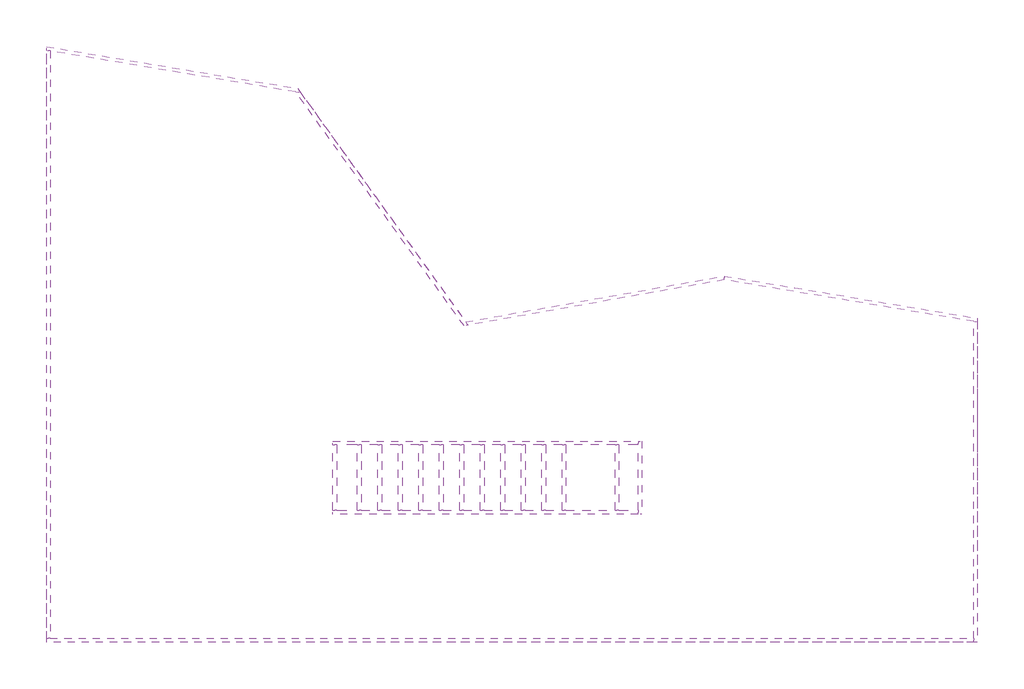
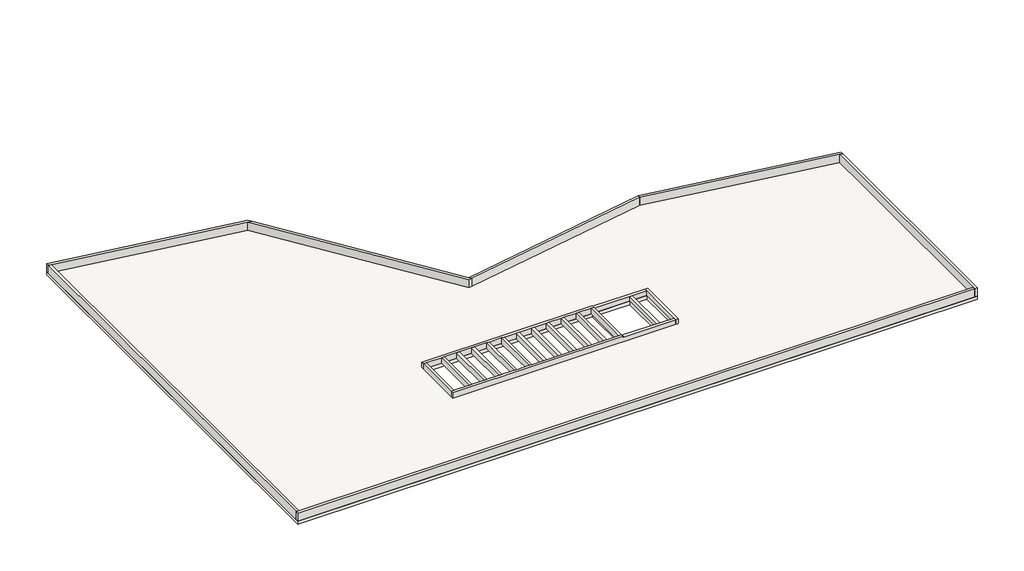
# One storey: 23 walls, 1 slab.
"""IFC4 building model written with IfcOpenShell, lengths in millimetres."""

from ifc_helpers import new_model, si_unit, frame, origin, place, context, project, spatial, polyline, outline, extrude, faceted_brep, element, save

model = new_model("IFC4")

# Units and contexts
model_context = context("Model", 3, world=origin())
ifc_project = project(units=[si_unit("LENGTHUNIT", "METRE", prefix="MILLI")], contexts=[model_context])

# Site, building, storey
site = spatial("IfcSite", under=ifc_project)
building = spatial("IfcBuilding", under=site)
storey = spatial("IfcBuildingStorey", under=building, Name="04_OG_OKFB_13,84", Elevation=13840.0)

# Slab
placement = place(None, origin())
element("IfcSlab", 1, ObjectType="5dki Decke Ortbeton 25cm C30/37_f", at=placement, inside=storey, context=model_context, shape_type="SweptSolid", body=[
    extrude(outline(polyline([(-129.9989953, 31855.7150729), (13359.8955383, 29603.0549033), (22383.5041721, 17069.4128529), (36259.9888873, 19532.5499737), (49863.9990833, 17260.8337794), (49863.9991105, -129.9989509), (-129.9989953, -129.9990284), (-129.9989953, 31855.7150729)]), holes=[polyline([(27641.9999883, 10442.0127204), (15367.0008797, 10442.0127204), (15367.0008797, 6960.0000464), (27641.9999883, 6960.0000464), (27641.9999883, 10442.0127204)]), polyline([(27891.9992024, 6990.0014141), (30391.5781103, 6990.0014141), (30391.5781103, 10412.0125176), (27891.9992024, 10412.0125176), (27891.9992024, 6990.0014141)]), polyline([(30635.8205887, 6960.0014903), (31641.9991143, 6960.0014903), (31641.9991143, 10412.0130303), (30635.8205887, 10412.0130303), (30635.8205887, 6960.0014903)])]), frame((0.0, 0.0, 16900.0), z_axis=(0.0, 0.0, 1.0), x_axis=(1.0, 0.0, 0.0)), (0.0, 0.0, 1.0), 250.0),
])

# Walls
element("IfcWall", 2, ObjectType="5dki Unterzug 20cm C25/30", at=placement, inside=storey, context=model_context, shape_type="Brep", body=[
    faceted_brep([(-130.0001888, 31652.9459223, 17150.0), (69.9998112, 31619.548179, 17150.0), (13245.710804, 29419.3531156, 17150.0), (13525.8286333, 29372.5765989, 17150.0), (13525.8286333, 29372.5765989, 17780.0), (13245.710804, 29419.3531156, 17780.0), (69.9998112, 31619.548179, 17780.0), (-130.0001888, 31652.9459223, 17780.0), (-130.0001888, 31855.7152722, 17150.0), (-130.0001888, 31855.7152722, 17780.0), (13359.8955383, 29603.0549033, 17780.0), (13359.8955383, 29603.0549033, 17150.0)], [[[0, 1, 2, 3, 4, 5, 6, 7]], [[8, 9, 10, 11]], [[3, 2, 1, 0, 8, 11]], [[7, 6, 5, 4, 10, 9]], [[4, 3, 11, 10]], [[0, 7, 9, 8]]]),
])
element("IfcWall", 3, ObjectType="5dki Unterzug 20cm C25/30", at=placement, inside=storey, context=model_context, shape_type="Brep", body=[
    faceted_brep([(13245.710804, 29419.3531156, 17150.0), (22294.6581946, 16850.5159542, 17150.0), (22294.6581946, 16850.5159542, 17780.0), (13245.710804, 29419.3531156, 17780.0), (13525.8286333, 29372.5765989, 17150.0), (13525.8286333, 29372.5765989, 17780.0), (22383.5041721, 17069.4128529, 17780.0), (22513.1740957, 16889.3034894, 17780.0), (22513.1740957, 16889.3034894, 17150.0), (22383.5041721, 17069.4128529, 17150.0)], [[[0, 1, 2, 3]], [[4, 5, 6, 7, 8, 9]], [[1, 0, 4, 9, 8]], [[3, 2, 7, 6, 5]], [[0, 3, 5, 4]], [[2, 1, 8, 7]]]),
])
element("IfcWall", 4, ObjectType="5dki Unterzug 20cm C25/30", at=placement, inside=storey, context=model_context, shape_type="SweptSolid", body=[
    extrude(outline(polyline([(36260.2920068, 19329.4774895), (22513.1740957, 16889.3034894), (22383.5041721, 17069.4128529), (36259.255712, 19532.4198889), (36260.2920068, 19329.4774895)])), frame((0.0, 0.0, 17150.0), z_axis=(0.0, 0.0, 1.0), x_axis=(1.0, 0.0, 0.0)), (0.0, 0.0, 1.0), 630.0),
])
element("IfcWall", 5, ObjectType="5dki Unterzug 20cm C25/30", at=placement, inside=storey, context=model_context, shape_type="Brep", body=[
    faceted_brep([(36260.2920068, 19329.4774895, 17150.0), (49663.9990837, 17091.2096558, 17150.0), (49863.9990837, 17057.8119126, 17150.0), (49863.9990837, 17057.8119126, 17780.0), (49663.9990837, 17091.2096558, 17780.0), (36260.2920068, 19329.4774895, 17780.0), (36259.255712, 19532.4198889, 17150.0), (36259.255712, 19532.4198889, 17780.0), (49863.9990834, 17260.5812626, 17780.0), (49863.9990834, 17260.5812626, 17150.0)], [[[0, 1, 2, 3, 4, 5]], [[6, 7, 8, 9]], [[2, 1, 0, 6, 9]], [[5, 4, 3, 8, 7]], [[0, 5, 7, 6]], [[3, 2, 9, 8]]]),
])
element("IfcWall", 6, ObjectType="5dki Unterzug 20cm C25/30", at=placement, inside=storey, context=model_context, shape_type="Brep", body=[
    faceted_brep([(49663.9990837, 17091.2096558, 17150.0), (49663.9991102, 70.0010491, 17150.0), (49663.9991105, -129.9989509, 17150.0), (49663.9991105, -129.9989509, 17780.0), (49663.9991102, 70.0010491, 17780.0), (49663.9990837, 17091.2096558, 17780.0), (49863.9990837, 17057.8119126, 17150.0), (49863.9990837, 17057.8119126, 17780.0), (49863.9991105, -129.9989509, 17780.0), (49863.9991105, -129.9989509, 17150.0)], [[[0, 1, 2, 3, 4, 5]], [[6, 7, 8, 9]], [[2, 1, 0, 6, 9]], [[5, 4, 3, 8, 7]], [[0, 5, 7, 6]], [[3, 2, 9, 8]]]),
])
element("IfcWall", 7, ObjectType="5dki Unterzug 20cm C25/30", at=placement, inside=storey, context=model_context, shape_type="Brep", body=[
    faceted_brep([(49663.9991102, 70.0010491, 17150.0), (69.9998112, 70.0010491, 17150.0), (-130.0001888, 70.0010491, 17150.0), (-130.0001888, 70.0010491, 17780.0), (69.9998112, 70.0010491, 17780.0), (49663.9991102, 70.0010491, 17780.0), (49663.9991105, -129.9989509, 17150.0), (49663.9991105, -129.9989509, 17780.0), (-130.0001888, -129.9989509, 17780.0), (-130.0001888, -129.9989509, 17150.0)], [[[0, 1, 2, 3, 4, 5]], [[6, 7, 8, 9]], [[2, 1, 0, 6, 9]], [[5, 4, 3, 8, 7]], [[0, 5, 7, 6]], [[3, 2, 9, 8]]]),
])
element("IfcWall", 8, ObjectType="5dki Unterzug 20cm C25/30", at=placement, inside=storey, context=model_context, shape_type="SweptSolid", body=[
    extrude(outline(polyline([(69.9998112, 31619.548179), (69.9998112, 70.0010491), (-130.0001888, 70.0010491), (-130.0001888, 31652.9459223), (69.9998112, 31619.548179)])), frame((0.0, 0.0, 17150.0), z_axis=(0.0, 0.0, 1.0), x_axis=(1.0, 0.0, 0.0)), (0.0, 0.0, 1.0), 630.0),
])
element("IfcWall", 9, ObjectType="5dki Überzug 20cm C30/37", at=placement, inside=storey, context=model_context, shape_type="Brep", body=[
    faceted_brep([(15242.0008797, 10462.0127204, 17150.0), (16566.9999827, 10462.0127204, 17150.0), (16766.9999827, 10462.0127204, 17150.0), (17666.9999827, 10462.0127204, 17150.0), (17866.9999827, 10462.0127204, 17150.0), (18766.9999827, 10462.0127204, 17150.0), (18966.9999827, 10462.0127204, 17150.0), (19866.9999827, 10462.0127204, 17150.0), (20066.9999827, 10462.0127204, 17150.0), (20966.9999827, 10462.0127204, 17150.0), (21166.9999827, 10462.0127204, 17150.0), (22066.9999827, 10462.0127204, 17150.0), (22266.9999827, 10462.0127204, 17150.0), (23166.9999827, 10462.0127204, 17150.0), (23366.9999827, 10462.0127204, 17150.0), (24266.9999827, 10462.0127204, 17150.0), (24466.9999827, 10462.0127204, 17150.0), (25366.9999827, 10462.0127204, 17150.0), (25566.9999827, 10462.0127204, 17150.0), (26466.9999827, 10462.0127204, 17150.0), (26666.9999827, 10462.0127204, 17150.0), (27566.9999827, 10462.0127204, 17150.0), (27766.9999827, 10462.0127204, 17150.0), (30401.9991143, 10462.0127204, 17150.0), (30601.9991143, 10462.0127204, 17150.0), (31641.9991143, 10462.0127204, 17150.0), (31641.9991143, 10462.0127204, 17530.0), (27766.9999827, 10462.0127204, 17530.0), (27766.9999827, 10462.0127204, 17580.0), (27566.9999827, 10462.0127204, 17580.0), (26666.9999827, 10462.0127204, 17580.0), (26466.9999827, 10462.0127204, 17580.0), (25566.9999827, 10462.0127204, 17580.0), (25366.9999827, 10462.0127204, 17580.0), (24466.9999827, 10462.0127204, 17580.0), (24266.9999827, 10462.0127204, 17580.0), (23366.9999827, 10462.0127204, 17580.0), (23166.9999827, 10462.0127204, 17580.0), (22266.9999827, 10462.0127204, 17580.0), (22066.9999827, 10462.0127204, 17580.0), (21166.9999827, 10462.0127204, 17580.0), (20966.9999827, 10462.0127204, 17580.0), (20066.9999827, 10462.0127204, 17580.0), (19866.9999827, 10462.0127204, 17580.0), (18966.9999827, 10462.0127204, 17580.0), (18766.9999827, 10462.0127204, 17580.0), (17866.9999827, 10462.0127204, 17580.0), (17666.9999827, 10462.0127204, 17580.0), (16766.9999827, 10462.0127204, 17580.0), (16566.9999827, 10462.0127204, 17580.0), (15442.0008797, 10462.0127204, 17580.0), (15242.0008797, 10462.0127204, 17580.0), (15242.0008797, 10662.0127204, 17150.0), (15242.0008797, 10662.0127204, 17580.0), (27766.9999827, 10662.0127204, 17580.0), (27766.9999827, 10662.0127204, 17530.0), (31641.9991143, 10662.0127204, 17530.0), (31641.9991143, 10662.0127204, 17150.0)], [[[0, 1, 2, 3, 4, 5, 6, 7, 8, 9, 10, 11, 12, 13, 14, 15, 16, 17, 18, 19, 20, 21, 22, 23, 24, 25, 26, 27, 28, 29, 30, 31, 32, 33, 34, 35, 36, 37, 38, 39, 40, 41, 42, 43, 44, 45, 46, 47, 48, 49, 50, 51]], [[52, 53, 54, 55, 56, 57]], [[0, 51, 53, 52]], [[26, 25, 57, 56]], [[25, 24, 23, 22, 21, 20, 19, 18, 17, 16, 15, 14, 13, 12, 11, 10, 9, 8, 7, 6, 5, 4, 3, 2, 1, 0, 52, 57]], [[27, 26, 56, 55]], [[51, 50, 49, 48, 47, 46, 45, 44, 43, 42, 41, 40, 39, 38, 37, 36, 35, 34, 33, 32, 31, 30, 29, 28, 54, 53]], [[28, 27, 55, 54]]]),
])
element("IfcWall", 10, ObjectType="5dki Überzug 20cm C30/37", at=placement, inside=storey, context=model_context, shape_type="Brep", body=[
    faceted_brep([(27566.9999827, 10462.0127204, 17580.0), (27566.9999827, 10462.0127204, 17150.0), (27566.9999827, 6940.0000311, 17150.0), (27566.9999827, 6940.0000311, 17580.0), (27766.9999827, 10462.0127204, 17150.0), (27766.9999827, 10462.0127204, 17530.0), (27766.9999827, 10462.0127204, 17580.0), (27766.9999827, 6940.0000311, 17580.0), (27766.9999827, 6940.0000311, 17530.0), (27766.9999827, 6940.0000311, 17150.0)], [[[0, 1, 2, 3]], [[4, 5, 6, 7, 8, 9]], [[2, 1, 4, 9]], [[0, 3, 7, 6]], [[0, 6, 5, 4, 1]], [[3, 2, 9, 8, 7]]]),
])
element("IfcWall", 11, ObjectType="5dki Überzug 20cm C30/37", at=placement, inside=storey, context=model_context, shape_type="Brep", body=[
    faceted_brep([(15242.0008797, 6940.0000311, 17150.0), (15242.0008797, 6940.0000311, 17580.0), (15442.0008797, 6940.0000311, 17580.0), (16566.9999827, 6940.0000311, 17580.0), (16766.9999827, 6940.0000311, 17580.0), (17666.9999827, 6940.0000311, 17580.0), (17866.9999827, 6940.0000311, 17580.0), (18766.9999827, 6940.0000311, 17580.0), (18966.9999827, 6940.0000311, 17580.0), (19866.9999827, 6940.0000311, 17580.0), (20066.9999827, 6940.0000311, 17580.0), (20966.9999827, 6940.0000311, 17580.0), (21166.9999827, 6940.0000311, 17580.0), (22066.9999827, 6940.0000311, 17580.0), (22266.9999827, 6940.0000311, 17580.0), (23166.9999827, 6940.0000311, 17580.0), (23366.9999827, 6940.0000311, 17580.0), (24266.9999827, 6940.0000311, 17580.0), (24466.9999827, 6940.0000311, 17580.0), (25366.9999827, 6940.0000311, 17580.0), (25566.9999827, 6940.0000311, 17580.0), (26466.9999827, 6940.0000311, 17580.0), (26666.9999827, 6940.0000311, 17580.0), (27566.9999827, 6940.0000311, 17580.0), (27766.9999827, 6940.0000311, 17580.0), (27766.9999827, 6940.0000311, 17530.0), (31641.9991143, 6940.0000311, 17530.0), (31641.9991143, 6940.0000311, 17150.0), (30601.9991143, 6940.0000311, 17150.0), (30401.9991143, 6940.0000311, 17150.0), (27766.9999827, 6940.0000311, 17150.0), (27566.9999827, 6940.0000311, 17150.0), (26666.9999827, 6940.0000311, 17150.0), (26466.9999827, 6940.0000311, 17150.0), (25566.9999827, 6940.0000311, 17150.0), (25366.9999827, 6940.0000311, 17150.0), (24466.9999827, 6940.0000311, 17150.0), (24266.9999827, 6940.0000311, 17150.0), (23366.9999827, 6940.0000311, 17150.0), (23166.9999827, 6940.0000311, 17150.0), (22266.9999827, 6940.0000311, 17150.0), (22066.9999827, 6940.0000311, 17150.0), (21166.9999827, 6940.0000311, 17150.0), (20966.9999827, 6940.0000311, 17150.0), (20066.9999827, 6940.0000311, 17150.0), (19866.9999827, 6940.0000311, 17150.0), (18966.9999827, 6940.0000311, 17150.0), (18766.9999827, 6940.0000311, 17150.0), (17866.9999827, 6940.0000311, 17150.0), (17666.9999827, 6940.0000311, 17150.0), (16766.9999827, 6940.0000311, 17150.0), (16566.9999827, 6940.0000311, 17150.0), (15242.0008797, 6740.0000311, 17150.0), (31641.9991143, 6740.0000311, 17150.0), (31641.9991143, 6740.0000311, 17530.0), (27766.9999827, 6740.0000311, 17530.0), (27766.9999827, 6740.0000311, 17580.0), (15242.0008797, 6740.0000311, 17580.0)], [[[0, 1, 2, 3, 4, 5, 6, 7, 8, 9, 10, 11, 12, 13, 14, 15, 16, 17, 18, 19, 20, 21, 22, 23, 24, 25, 26, 27, 28, 29, 30, 31, 32, 33, 34, 35, 36, 37, 38, 39, 40, 41, 42, 43, 44, 45, 46, 47, 48, 49, 50, 51]], [[52, 53, 54, 55, 56, 57]], [[1, 0, 52, 57]], [[0, 51, 50, 49, 48, 47, 46, 45, 44, 43, 42, 41, 40, 39, 38, 37, 36, 35, 34, 33, 32, 31, 30, 29, 28, 27, 53, 52]], [[24, 23, 22, 21, 20, 19, 18, 17, 16, 15, 14, 13, 12, 11, 10, 9, 8, 7, 6, 5, 4, 3, 2, 1, 57, 56]], [[26, 25, 55, 54]], [[27, 26, 54, 53]], [[25, 24, 56, 55]]]),
])
element("IfcWall", 12, ObjectType="5dki Überzug 20cm C30/37", at=placement, inside=storey, context=model_context, shape_type="Brep", body=[
    faceted_brep([(15442.0008797, 6940.0000311, 16900.0), (15442.0008797, 10462.0127204, 16900.0), (15442.0008797, 10462.0127204, 17580.0), (15442.0008797, 6940.0000311, 17580.0), (15242.0008797, 6940.0000311, 16900.0), (15242.0008797, 6940.0000311, 17150.0), (15242.0008797, 6940.0000311, 17580.0), (15242.0008797, 10462.0127204, 17580.0), (15242.0008797, 10462.0127204, 17150.0), (15242.0008797, 10462.0127204, 16900.0)], [[[0, 1, 2, 3]], [[4, 5, 6, 7, 8, 9]], [[1, 0, 4, 9]], [[3, 2, 7, 6]], [[2, 1, 9, 8, 7]], [[0, 3, 6, 5, 4]]]),
])
element("IfcWall", 13, ObjectType="5dki Überzug 20cm C30/37", at=placement, inside=storey, context=model_context, shape_type="Brep", body=[
    faceted_brep([(31641.9991143, 10662.0127204, 17150.0), (31641.9991143, 10462.0127204, 17150.0), (31641.9991143, 6940.0000311, 17150.0), (31641.9991143, 6740.0000311, 17150.0), (31641.9991143, 6740.0000311, 17530.0), (31641.9991143, 6940.0000311, 17530.0), (31641.9991143, 10462.0127204, 17530.0), (31641.9991143, 10662.0127204, 17530.0), (31841.9991143, 10662.0127204, 17150.0), (31841.9991143, 10662.0127204, 17530.0), (31841.9991143, 6740.0000311, 17530.0), (31841.9991143, 6740.0000311, 17150.0)], [[[0, 1, 2, 3, 4, 5, 6, 7]], [[8, 9, 10, 11]], [[4, 3, 11, 10]], [[0, 7, 9, 8]], [[3, 2, 1, 0, 8, 11]], [[7, 6, 5, 4, 10, 9]]]),
])
element("IfcWall", 14, ObjectType="5dki Überzug 20cm C30/37", at=placement, inside=storey, context=model_context, shape_type="SweptSolid", body=[
    extrude(outline(polyline([(30401.9991143, 6940.0000311), (30401.9991143, 10462.0127204), (30601.9991143, 10462.0127204), (30601.9991143, 6940.0000311), (30401.9991143, 6940.0000311)])), frame((0.0, 0.0, 17150.0), z_axis=(0.0, 0.0, 1.0), x_axis=(1.0, 0.0, 0.0)), (0.0, 0.0, 1.0), 350.0),
])
element("IfcWall", 15, ObjectType="5dki Überzug 20cm C30/37", at=placement, inside=storey, context=model_context, shape_type="SweptSolid", body=[
    extrude(outline(polyline([(26466.9999827, 6940.0000311), (26466.9999827, 10462.0127204), (26666.9999827, 10462.0127204), (26666.9999827, 6940.0000311), (26466.9999827, 6940.0000311)])), frame((0.0, 0.0, 17150.0), z_axis=(0.0, 0.0, 1.0), x_axis=(1.0, 0.0, 0.0)), (0.0, 0.0, 1.0), 430.0),
])
element("IfcWall", 16, ObjectType="5dki Überzug 20cm C30/37", at=placement, inside=storey, context=model_context, shape_type="SweptSolid", body=[
    extrude(outline(polyline([(25366.9999827, 6940.0000311), (25366.9999827, 10462.0127204), (25566.9999827, 10462.0127204), (25566.9999827, 6940.0000311), (25366.9999827, 6940.0000311)])), frame((0.0, 0.0, 17150.0), z_axis=(0.0, 0.0, 1.0), x_axis=(1.0, 0.0, 0.0)), (0.0, 0.0, 1.0), 430.0),
])
element("IfcWall", 17, ObjectType="5dki Überzug 20cm C30/37", at=placement, inside=storey, context=model_context, shape_type="SweptSolid", body=[
    extrude(outline(polyline([(24266.9999827, 6940.0000311), (24266.9999827, 10462.0127204), (24466.9999827, 10462.0127204), (24466.9999827, 6940.0000311), (24266.9999827, 6940.0000311)])), frame((0.0, 0.0, 17150.0), z_axis=(0.0, 0.0, 1.0), x_axis=(1.0, 0.0, 0.0)), (0.0, 0.0, 1.0), 430.0),
])
element("IfcWall", 18, ObjectType="5dki Überzug 20cm C30/37", at=placement, inside=storey, context=model_context, shape_type="SweptSolid", body=[
    extrude(outline(polyline([(23166.9999827, 6940.0000311), (23166.9999827, 10462.0127204), (23366.9999827, 10462.0127204), (23366.9999827, 6940.0000311), (23166.9999827, 6940.0000311)])), frame((0.0, 0.0, 17150.0), z_axis=(0.0, 0.0, 1.0), x_axis=(1.0, 0.0, 0.0)), (0.0, 0.0, 1.0), 430.0),
])
element("IfcWall", 19, ObjectType="5dki Überzug 20cm C30/37", at=placement, inside=storey, context=model_context, shape_type="SweptSolid", body=[
    extrude(outline(polyline([(22066.9999827, 6940.0000311), (22066.9999827, 10462.0127204), (22266.9999827, 10462.0127204), (22266.9999827, 6940.0000311), (22066.9999827, 6940.0000311)])), frame((0.0, 0.0, 17150.0), z_axis=(0.0, 0.0, 1.0), x_axis=(1.0, 0.0, 0.0)), (0.0, 0.0, 1.0), 430.0),
])
element("IfcWall", 20, ObjectType="5dki Überzug 20cm C30/37", at=placement, inside=storey, context=model_context, shape_type="SweptSolid", body=[
    extrude(outline(polyline([(20966.9999827, 6940.0000311), (20966.9999827, 10462.0127204), (21166.9999827, 10462.0127204), (21166.9999827, 6940.0000311), (20966.9999827, 6940.0000311)])), frame((0.0, 0.0, 17150.0), z_axis=(0.0, 0.0, 1.0), x_axis=(1.0, 0.0, 0.0)), (0.0, 0.0, 1.0), 430.0),
])
element("IfcWall", 21, ObjectType="5dki Überzug 20cm C30/37", at=placement, inside=storey, context=model_context, shape_type="SweptSolid", body=[
    extrude(outline(polyline([(19866.9999827, 6940.0000311), (19866.9999827, 10462.0127204), (20066.9999827, 10462.0127204), (20066.9999827, 6940.0000311), (19866.9999827, 6940.0000311)])), frame((0.0, 0.0, 17150.0), z_axis=(0.0, 0.0, 1.0), x_axis=(1.0, 0.0, 0.0)), (0.0, 0.0, 1.0), 430.0),
])
element("IfcWall", 22, ObjectType="5dki Überzug 20cm C30/37", at=placement, inside=storey, context=model_context, shape_type="SweptSolid", body=[
    extrude(outline(polyline([(18766.9999827, 6940.0000311), (18766.9999827, 10462.0127204), (18966.9999827, 10462.0127204), (18966.9999827, 6940.0000311), (18766.9999827, 6940.0000311)])), frame((0.0, 0.0, 17150.0), z_axis=(0.0, 0.0, 1.0), x_axis=(1.0, 0.0, 0.0)), (0.0, 0.0, 1.0), 430.0),
])
element("IfcWall", 23, ObjectType="5dki Überzug 20cm C30/37", at=placement, inside=storey, context=model_context, shape_type="SweptSolid", body=[
    extrude(outline(polyline([(17666.9999827, 6940.0000311), (17666.9999827, 10462.0127204), (17866.9999827, 10462.0127204), (17866.9999827, 6940.0000311), (17666.9999827, 6940.0000311)])), frame((0.0, 0.0, 17150.0), z_axis=(0.0, 0.0, 1.0), x_axis=(1.0, 0.0, 0.0)), (0.0, 0.0, 1.0), 430.0),
])
element("IfcWall", 24, ObjectType="5dki Überzug 20cm C30/37", at=placement, inside=storey, context=model_context, shape_type="SweptSolid", body=[
    extrude(outline(polyline([(16566.9999827, 6940.0000311), (16566.9999827, 10462.0127204), (16766.9999827, 10462.0127204), (16766.9999827, 6940.0000311), (16566.9999827, 6940.0000311)])), frame((0.0, 0.0, 17150.0), z_axis=(0.0, 0.0, 1.0), x_axis=(1.0, 0.0, 0.0)), (0.0, 0.0, 1.0), 430.0),
])

save(model, "model.ifc")

# Revit data of these elements
# Type "5dki Decke Ortbeton 25cm C30/37_f"
#   cpiComponentType = "Slab"
#   cpiFitMatchKey = ""
#   5d Materialgüte = "C30/37"
#   Function = 0
#   5dki WU = no
#   Layers, outside or top first: 0.250 m "5d Beton - Stahlbeton" (function 1)
# Type "5dki Unterzug 20cm C25/30"
#   Type Comments = ""
#   Description = ""
#   cpiComponentType = "Beam"
#   cpiFitMatchKey = "5D-KI-STB-OB-TR-UZ"
#   5d Materialgüte = "C25/30"
#   Filter Tragend / Nichttragend = yes
#   5dki WU = no
#   Layers, outside or top first: 0.200 m "5d Beton - Stahlbeton" (function 1)
# Type "5dki Überzug 20cm C30/37"
#   Type Comments = ""
#   Description = ""
#   cpiComponentType = "Beam"
#   cpiFitMatchKey = "5D-KI-STB-OB-TR-UEZ"
#   5d Materialgüte = "C30/37"
#   Filter Tragend / Nichttragend = yes
#   Layers, outside or top first: 0.200 m "5d Beton - Stahlbeton" (function 1)
# Element 1 (IfcSlab, "5dki Decke Ortbeton 25cm C30/37_f")
#   000_080_030_Geschoß = "04_OG"
#   built-in parameter 1001955 = 2.97613 (stored number, unit not read)
#   Height Offset From Level = 0.000 m
#   built-in parameter 1001954 = 1
#   Phase Created = Neu
#   Materials on its faces: "5d Beton - Stahlbeton"
# Elements 2, 3, 4, 5, 6, 7, 8 (IfcWall, "5dki Unterzug 20cm C25/30")
#   Comments = ""
#   000_080_030_Geschoß = "04_OG"
#   Top Offset = 0.000 m
#   Base Offset = 0.000 m
#   wall height = 0.630 m
#   Phase Created = Neu
#   Base Constraint = 04_OG_OKRD_17,15
#   Top Constraint = 05_DA_ATOK_17,78
#   Materials on its faces: "5d Beton - Stahlbeton"
# Elements 9, 10, 11, 13, 15, 16, 17, 18, 19, 20, 21, 22, 23, 24 (IfcWall, "5dki Überzug 20cm C30/37")
#   Comments = ""
#   000_080_030_Geschoß = "04_OG"
#   Top Offset = 0.000 m
#   Base Offset = 0.000 m
#   wall height = 0.430 m
#   Phase Created = Neu
#   Base Constraint = 04_OG_OKRD_17,15
#   Top Constraint = 05_DA_UKRD_17,58
#   Materials on its faces: "5d Beton - Stahlbeton"
# Element 12 (IfcWall, "5dki Überzug 20cm C30/37")
#   Comments = ""
#   000_080_030_Geschoß = "04_OG"
#   Top Offset = 0.000 m
#   Base Offset = 0.000 m
#   wall height = 0.680 m
#   Phase Created = Neu
#   Base Constraint = 04_OG_UKRD_16,90
#   Top Constraint = 05_DA_UKRD_17,58
#   Materials on its faces: "5d Beton - Stahlbeton"
# Element 14 (IfcWall, "5dki Überzug 20cm C30/37")
#   Comments = ""
#   000_080_030_Geschoß = "04_OG"
#   Top Offset = 0.000 m
#   Base Offset = 0.000 m
#   wall height = 0.350 m
#   Phase Created = Neu
#   Base Constraint = 04_OG_OKRD_17,15
#   Top Constraint = 05_DA_DAEM_17,50
#   Materials on its faces: "5d Beton - Stahlbeton"
# Materials
#   "5d Beton - Stahlbeton": class "5dki", colour RGB 200 200 200, transparency 0, Cost = 0
